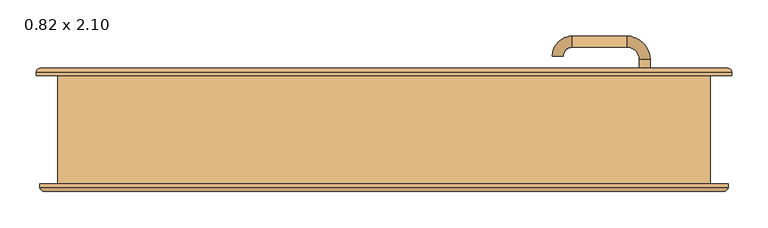
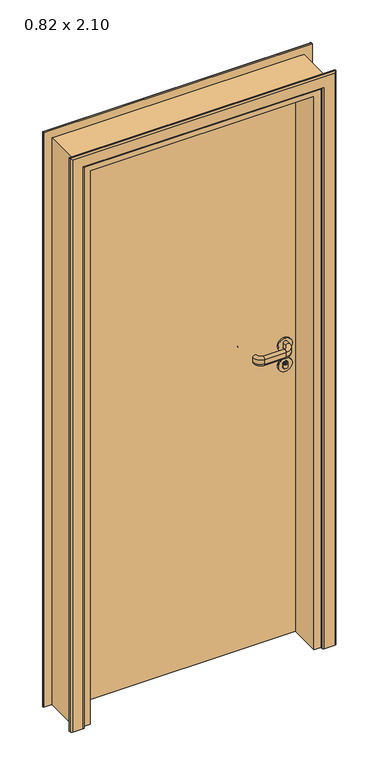
"""IFC4 building model written with IfcOpenShell, lengths in millimetres: door geometry, CC_PORTA ABRIR_1 FOLHA LISA : 0.82 x 2.10."""

from ifc_helpers import new_model, si_unit, point, frame, frame_2d, origin, origin_with_axes, place, context, project, spatial, polyline, circle_curve, ellipse_curve, trimmed, segment, composite_curve, outline, extrude, faceted_brep, source, transform, mapped, element, save
from ifc_brep_helpers import plane_surface, cylinder_surface, revolved_surface, advanced_brep


def door_0_82_x_2_10_9ce577dd(model_context):
    return source(origin(), model_context, "Body", "SolidModel", [
        advanced_brep(
        [(352.5, 40.0, 1091.5062746), (352.5, 40.0, 1108.3826844), (367.5, 40.0, 1108.3826844), (367.5, 40.0, 1091.5062746), (367.5, 18.0, 1108.3826844), (367.5, 18.0, 1091.5062746), (352.5, 18.0, 1091.5062746), (352.5, 18.0, 1108.3826844), (335.0, -14.5, 1108.3826844), (260.0, -14.5, 1108.3826844), (260.0, -14.5, 1091.5062746), (335.0, -14.5, 1091.5062746), (335.0, 0.5, 1091.5062746), (260.0, 0.5, 1091.5062746), (260.0, 0.5, 1108.3826844), (335.0, 0.5, 1108.3826844), (247.5, 13.0, 1091.5062746), (232.5, 13.0, 1091.5062746), (232.5, 13.0, 1108.3826844), (247.5, 13.0, 1108.3826844)],
        [
            (0, 1),
            (1, 2, circle_curve(frame((360.0, 40.0, 1108.3826844), z_axis=(0.0, 1.0, 0.0), x_axis=(0.0, 0.0, 1.0)), 7.5)),
            (2, 3),
            (3, 0, circle_curve(frame((360.0, 40.0, 1091.5062746), z_axis=(0.0, 1.0, 0.0), x_axis=(0.0, 0.0, 1.0)), 7.5)),
            (2, 4),
            (4, 5),
            (5, 3),
            (0, 6),
            (6, 7),
            (7, 1),
            (8, 9),
            (9, 10),
            (10, 11),
            (11, 8),
            (12, 13),
            (13, 14),
            (14, 15),
            (15, 12),
            (5, 6, circle_curve(frame((360.0, 18.0, 1091.5062746), z_axis=(0.0, 1.0, 0.0), x_axis=(0.0, 0.0, 1.0)), 7.5)),
            (7, 4, circle_curve(frame((360.0, 18.0, 1108.3826844), z_axis=(0.0, 1.0, 0.0), x_axis=(0.0, 0.0, 1.0)), 7.5)),
            (10, 13, circle_curve(frame((260.0, -7.0, 1091.5062746), z_axis=(1.0, 0.0, 0.0), x_axis=(0.0, 0.0, 1.0)), 7.5)),
            (12, 11, circle_curve(frame((335.0, -7.0, 1091.5062746), z_axis=(-1.0, 0.0, 0.0), x_axis=(0.0, 0.0, 1.0)), 7.5)),
            (14, 9, circle_curve(frame((260.0, -7.0, 1108.3826844), z_axis=(1.0, 0.0, 0.0), x_axis=(0.0, 0.0, 1.0)), 7.5)),
            (8, 15, circle_curve(frame((335.0, -7.0, 1108.3826844), z_axis=(-1.0, 0.0, 0.0), x_axis=(0.0, 0.0, 1.0)), 7.5)),
            (12, 6, circle_curve(frame((335.0, 18.0, 1091.5062746), z_axis=(0.0, 0.0, 1.0), x_axis=(1.0, 0.0, 0.0)), 17.5)),
            (5, 11, circle_curve(frame((335.0, 18.0, 1091.5062746), z_axis=(0.0, 0.0, -1.0), x_axis=(1.0, 0.0, 0.0)), 32.5)),
            (4, 8, circle_curve(frame((335.0, 18.0, 1108.3826844), z_axis=(0.0, 0.0, -1.0), x_axis=(1.0, 0.0, 0.0)), 32.5)),
            (7, 15, circle_curve(frame((335.0, 18.0, 1108.3826844), z_axis=(0.0, 0.0, -1.0), x_axis=(1.0, 0.0, 0.0)), 17.5)),
            (16, 17, circle_curve(frame((240.0, 13.0, 1091.5062746), z_axis=(0.0, 1.0, 0.0), x_axis=(0.0, 0.0, 1.0)), 7.5)),
            (17, 18),
            (18, 19, circle_curve(frame((240.0, 13.0, 1108.3826844), z_axis=(0.0, 1.0, 0.0), x_axis=(0.0, 0.0, 1.0)), 7.5)),
            (19, 16),
            (16, 13, circle_curve(frame((260.0, 13.0, 1091.5062746), z_axis=(0.0, 0.0, 1.0), x_axis=(0.0, -1.0, 0.0)), 12.5)),
            (10, 17, circle_curve(frame((260.0, 13.0, 1091.5062746), z_axis=(0.0, 0.0, -1.0), x_axis=(0.0, -1.0, 0.0)), 27.5)),
            (9, 18, circle_curve(frame((260.0, 13.0, 1108.3826844), z_axis=(0.0, 0.0, -1.0), x_axis=(0.0, -1.0, 0.0)), 27.5)),
            (14, 19, circle_curve(frame((260.0, 13.0, 1108.3826844), z_axis=(0.0, 0.0, -1.0), x_axis=(0.0, -1.0, 0.0)), 12.5)),
        ],
        [
            plane_surface(frame((360.0, 40.0, 1099.9444795), z_axis=(0.0, 1.0, 0.0), x_axis=(0.0, 0.0, 1.0))),
            plane_surface(frame((367.5, 40.0, 1091.5062746), z_axis=(1.0, 0.0, 0.0), x_axis=(0.0, -1.0, 0.0))),
            plane_surface(frame((352.5, 40.0, 1108.3826844), z_axis=(-1.0, 0.0, 0.0), x_axis=(0.0, -1.0, 0.0))),
            plane_surface(frame((335.0, -14.5, 1091.5062746), z_axis=(0.0, -1.0, 0.0), x_axis=(-1.0, 0.0, 0.0))),
            plane_surface(frame((335.0, 0.5, 1108.3826844), z_axis=(0.0, 1.0, 0.0), x_axis=(-1.0, 0.0, 0.0))),
            cylinder_surface(frame((360.0, 40.0, 1091.5062746), z_axis=(0.0, 1.0, 0.0), x_axis=(0.0, 0.0, 1.0)), 7.5),
            cylinder_surface(frame((360.0, 40.0, 1108.3826844), z_axis=(0.0, 1.0, 0.0), x_axis=(0.0, 0.0, 1.0)), 7.5),
            cylinder_surface(frame((335.0, -7.0, 1091.5062746), z_axis=(1.0, 0.0, 0.0), x_axis=(0.0, 0.0, 1.0)), 7.5),
            cylinder_surface(frame((335.0, -7.0, 1108.3826844), z_axis=(1.0, 0.0, 0.0), x_axis=(0.0, 0.0, 1.0)), 7.5),
            revolved_surface(trimmed(ellipse_curve(frame((360.0, 18.0, 1091.5062746), z_axis=(0.0, -1.0, 0.0), x_axis=(0.0, 0.0, 1.0)), 7.5, 7.5), [point((352.5, 18.0, 1091.5062746))], [point((367.5, 18.0, 1091.5062746))], True, "CARTESIAN"), (335.0, 18.0, 1099.9444795), (0.0, 0.0, 1.0)),
            cylinder_surface(frame((335.0, 18.0, 1099.9444795), z_axis=(0.0, 0.0, 1.0), x_axis=(1.0, 0.0, 0.0)), 32.5),
            revolved_surface(trimmed(ellipse_curve(frame((360.0, 18.0, 1108.3826844), z_axis=(0.0, -1.0, 0.0), x_axis=(0.0, 0.0, 1.0)), 7.5, 7.5), [point((367.5, 18.0, 1108.3826844))], [point((352.5, 18.0, 1108.3826844))], True, "CARTESIAN"), (335.0, 18.0, 1099.9444795), (0.0, 0.0, 1.0)),
            revolved_surface(polyline([(352.5, 18.0, 1108.3826844), (352.5, 18.0, 1091.5062746)]), (335.0, 18.0, 1099.9444795), (0.0, 0.0, 1.0)),
            plane_surface(frame((240.0, 13.0, 1099.9444795), z_axis=(0.0, 1.0, 0.0), x_axis=(0.0, 0.0, 1.0))),
            revolved_surface(trimmed(ellipse_curve(frame((260.0, -7.0, 1091.5062746), z_axis=(-1.0, 0.0, 0.0), x_axis=(0.0, 0.0, 1.0)), 7.5, 7.5), [point((260.0, 0.5, 1091.5062746))], [point((260.0, -14.5, 1091.5062746))], True, "CARTESIAN"), (260.0, 13.0, 1099.9444795), (0.0, 0.0, 1.0)),
            cylinder_surface(frame((260.0, 13.0, 1099.9444795), z_axis=(0.0, 0.0, 1.0), x_axis=(0.0, -1.0, 0.0)), 27.5),
            revolved_surface(trimmed(ellipse_curve(frame((260.0, -7.0, 1108.3826844), z_axis=(-1.0, 0.0, 0.0), x_axis=(0.0, 0.0, 1.0)), 7.5, 7.5), [point((260.0, -14.5, 1108.3826844))], [point((260.0, 0.5, 1108.3826844))], True, "CARTESIAN"), (260.0, 13.0, 1099.9444795), (0.0, 0.0, 1.0)),
            revolved_surface(polyline([(260.0, 0.5, 1108.3826844), (260.0, 0.5, 1091.5062746)]), (260.0, 13.0, 1099.9444795), (0.0, 0.0, 1.0)),
        ],
        [
            (0, [[1, 2, 3, 4]]),
            (1, [[5, 6, 7, -3]]),
            (2, [[8, 9, 10, -1]]),
            (3, [[11, 12, 13, 14]]),
            (4, [[15, 16, 17, 18]]),
            (5, [[-7, 19, -8, -4]]),
            (6, [[-10, 20, -5, -2]]),
            (7, [[-13, 21, -15, 22]]),
            (8, [[-17, 23, -11, 24]]),
            (9, [[-22, 25, -19, 26]]),
            (10, [[-14, -26, -6, 27]]),
            (11, [[-24, -27, -20, 28]]),
            (12, [[-18, -28, -9, -25]]),
            (13, [[29, 30, 31, 32]]),
            (14, [[-29, 33, -21, 34]]),
            (15, [[-30, -34, -12, 35]]),
            (16, [[-31, -35, -23, 36]]),
            (17, [[-32, -36, -16, -33]]),
        ],
    ),
        extrude(outline(polyline([(361.0, 40.0), (361.0, 30.9), (359.0, 30.9), (359.0, 40.0), (361.0, 40.0)])), frame((0.0, 0.0, 1027.9555433), z_axis=(0.0, 0.0, 1.0), x_axis=(1.0, 0.0, 0.0)), (0.0, 0.0, 1.0), 7.8071257),
        extrude(outline(composite_curve([segment(trimmed(circle_curve(frame_2d((1031.5611613, 360.0)), 5.0), [point((1036.5611613, 360.0))], [point((1026.5611613, 360.0))], False, "CARTESIAN"), True, "CONTINUOUS"), segment(trimmed(circle_curve(frame_2d((1031.5611613, 360.0)), 5.0), [point((1026.5611613, 360.0))], [point((1036.5611613, 360.0))], False, "CARTESIAN"), True, "CONTINUOUS")], self_intersect=False), holes=[polyline([(1035.7626689, 361.0), (1027.9555433, 361.0), (1027.9555433, 359.0), (1035.7626689, 359.0), (1035.7626689, 361.0)])]), frame((0.0, 30.0, 0.0), z_axis=(0.0, 1.0, 0.0), x_axis=(0.0, 0.0, 1.0)), (0.0, 0.0, 1.0), 10.0),
        extrude(outline(composite_curve([segment(polyline([(1033.4817325, 352.5), (1016.4817325, 352.5)]), True, "CONTINUOUS"), segment(trimmed(circle_curve(frame_2d((1016.4817325, 356.5)), 4.0), [point((1016.4817325, 352.5))], [point((1012.4817325, 356.5))], False, "CARTESIAN"), True, "CONTINUOUS"), segment(polyline([(1012.4817325, 356.5), (1012.4817325, 363.5)]), True, "CONTINUOUS"), segment(trimmed(circle_curve(frame_2d((1016.4817325, 363.5)), 4.0), [point((1012.4817325, 363.5))], [point((1016.4817325, 367.5))], False, "CARTESIAN"), True, "CONTINUOUS"), segment(polyline([(1016.4817325, 367.5), (1033.4817325, 367.5)]), True, "CONTINUOUS"), segment(trimmed(circle_curve(frame_2d((1033.4817325, 363.5)), 4.0), [point((1033.4817325, 367.5))], [point((1037.4817325, 363.5))], False, "CARTESIAN"), True, "CONTINUOUS"), segment(polyline([(1037.4817325, 363.5), (1037.4817325, 356.5)]), True, "CONTINUOUS"), segment(trimmed(circle_curve(frame_2d((1033.4817325, 356.5)), 4.0), [point((1037.4817325, 356.5))], [point((1033.4817325, 352.5))], False, "CARTESIAN"), True, "CONTINUOUS")], self_intersect=False)), frame((0.0, 31.0, 0.0), z_axis=(0.0, 1.0, 0.0), x_axis=(0.0, 0.0, 1.0)), (0.0, 0.0, 1.0), 9.0),
        extrude(outline(composite_curve([segment(trimmed(circle_curve(frame_2d((1099.9444795, 360.0)), 25.0), [point((1124.9444795, 360.0))], [point((1074.9444795, 360.0))], False, "CARTESIAN"), True, "CONTINUOUS"), segment(trimmed(circle_curve(frame_2d((1099.9444795, 360.0)), 25.0), [point((1074.9444795, 360.0))], [point((1124.9444795, 360.0))], False, "CARTESIAN"), True, "CONTINUOUS")], self_intersect=False)), frame((0.0, 34.0, 0.0), z_axis=(0.0, 1.0, 0.0), x_axis=(0.0, 0.0, 1.0)), (0.0, 0.0, 1.0), 6.0),
        extrude(outline(composite_curve([segment(trimmed(circle_curve(frame_2d((1024.9444795, 360.0)), 25.0), [point((1049.9444795, 360.0))], [point((999.9444795, 360.0))], False, "CARTESIAN"), True, "CONTINUOUS"), segment(trimmed(circle_curve(frame_2d((1024.9444795, 360.0)), 25.0), [point((999.9444795, 360.0))], [point((1049.9444795, 360.0))], False, "CARTESIAN"), True, "CONTINUOUS")], self_intersect=False), holes=[composite_curve([segment(trimmed(circle_curve(frame_2d((1033.4817325, 363.5)), 4.0), [point((1037.4817325, 363.5))], [point((1033.4817325, 367.5))], True, "CARTESIAN"), True, "CONTINUOUS"), segment(polyline([(1033.4817325, 367.5), (1016.4817325, 367.5)]), True, "CONTINUOUS"), segment(trimmed(circle_curve(frame_2d((1016.4817325, 363.5)), 4.0), [point((1016.4817325, 367.5))], [point((1012.4817325, 363.5))], True, "CARTESIAN"), True, "CONTINUOUS"), segment(polyline([(1012.4817325, 363.5), (1012.4817325, 356.5)]), True, "CONTINUOUS"), segment(trimmed(circle_curve(frame_2d((1016.4817325, 356.5)), 4.0), [point((1012.4817325, 356.5))], [point((1016.4817325, 352.5))], True, "CARTESIAN"), True, "CONTINUOUS"), segment(polyline([(1016.4817325, 352.5), (1033.4817325, 352.5)]), True, "CONTINUOUS"), segment(trimmed(circle_curve(frame_2d((1033.4817325, 356.5)), 4.0), [point((1033.4817325, 352.5))], [point((1037.4817325, 356.5))], True, "CARTESIAN"), True, "CONTINUOUS"), segment(polyline([(1037.4817325, 356.5), (1037.4817325, 363.5)]), True, "CONTINUOUS")], self_intersect=False)]), frame((0.0, 34.0, 0.0), z_axis=(0.0, 1.0, 0.0), x_axis=(0.0, 0.0, 1.0)), (0.0, 0.0, 1.0), 6.0),
        extrude(outline(polyline([(361.0, 84.1), (361.0, 75.0), (359.0, 75.0), (359.0, 84.1), (361.0, 84.1)])), frame((0.0, 0.0, 1027.9555433), z_axis=(0.0, 0.0, 1.0), x_axis=(1.0, 0.0, 0.0)), (0.0, 0.0, 1.0), 7.8071257),
        advanced_brep(
        [(360.0, 85.0, 1036.5611613), (360.0, 85.0, 1026.5611613), (361.0, 85.0, 1035.7626689), (359.0, 85.0, 1035.7626689), (359.0, 85.0, 1027.9555433), (361.0, 85.0, 1027.9555433), (360.0, 75.0, 1049.9444795), (360.0, 75.0, 999.9444795), (360.0, 84.0, 1026.5611613), (360.0, 84.0, 1036.5611613), (361.0, 84.0, 1027.9555433), (361.0, 84.0, 1035.7626689), (359.0, 84.0, 1027.9555433), (359.0, 84.0, 1035.7626689), (352.5, 84.0, 1033.4817325), (356.5, 84.0, 1037.4817325), (363.5, 84.0, 1037.4817325), (367.5, 84.0, 1033.4817325), (367.5, 84.0, 1016.4817325), (363.5, 84.0, 1012.4817325), (356.5, 84.0, 1012.4817325), (352.5, 84.0, 1016.4817325), (352.5, 81.0, 1016.4817325), (352.5, 81.0, 1033.4817325), (356.5, 81.0, 1012.4817325), (363.5, 81.0, 1012.4817325), (367.5, 81.0, 1016.4817325), (367.5, 81.0, 1033.4817325), (363.5, 81.0, 1037.4817325), (356.5, 81.0, 1037.4817325), (360.0, 81.0, 1049.9444795), (360.0, 81.0, 999.9444795)],
        [
            (0, 1, circle_curve(frame((360.0, 85.0, 1031.5611613), z_axis=(0.0, 1.0, 0.0), x_axis=(0.0, 0.0, -1.0)), 5.0)),
            (1, 0, circle_curve(frame((360.0, 85.0, 1031.5611613), z_axis=(0.0, 1.0, 0.0), x_axis=(0.0, 0.0, -1.0)), 5.0)),
            (2, 3),
            (3, 4),
            (4, 5),
            (5, 2),
            (6, 7, circle_curve(frame((360.0, 75.0, 1024.9444795), z_axis=(0.0, -1.0, 0.0), x_axis=(0.0, 0.0, -1.0)), 25.0)),
            (7, 6, circle_curve(frame((360.0, 75.0, 1024.9444795), z_axis=(0.0, -1.0, 0.0), x_axis=(0.0, 0.0, -1.0)), 25.0)),
            (1, 8),
            (8, 9, circle_curve(frame((360.0, 84.0, 1031.5611613), z_axis=(0.0, 1.0, 0.0), x_axis=(0.0, 0.0, -1.0)), 5.0)),
            (9, 0),
            (9, 8, circle_curve(frame((360.0, 84.0, 1031.5611613), z_axis=(0.0, 1.0, 0.0), x_axis=(0.0, 0.0, -1.0)), 5.0)),
            (5, 10),
            (10, 11),
            (11, 2),
            (4, 12),
            (12, 10),
            (3, 13),
            (13, 12),
            (11, 13),
            (14, 15, circle_curve(frame((356.5, 84.0, 1033.4817325), z_axis=(0.0, 1.0, 0.0), x_axis=(0.0, 0.0, -1.0)), 4.0)),
            (15, 16),
            (16, 17, circle_curve(frame((363.5, 84.0, 1033.4817325), z_axis=(0.0, 1.0, 0.0), x_axis=(0.0, 0.0, -1.0)), 4.0)),
            (17, 18),
            (18, 19, circle_curve(frame((363.5, 84.0, 1016.4817325), z_axis=(0.0, 1.0, 0.0), x_axis=(0.0, 0.0, -1.0)), 4.0)),
            (19, 20),
            (20, 21, circle_curve(frame((356.5, 84.0, 1016.4817325), z_axis=(0.0, 1.0, 0.0), x_axis=(0.0, 0.0, -1.0)), 4.0)),
            (21, 14),
            (21, 22),
            (22, 23),
            (23, 14),
            (20, 24),
            (24, 22, circle_curve(frame((356.5, 81.0, 1016.4817325), z_axis=(0.0, 1.0, 0.0), x_axis=(0.0, 0.0, -1.0)), 4.0)),
            (19, 25),
            (25, 24),
            (18, 26),
            (26, 25, circle_curve(frame((363.5, 81.0, 1016.4817325), z_axis=(0.0, 1.0, 0.0), x_axis=(0.0, 0.0, -1.0)), 4.0)),
            (17, 27),
            (27, 26),
            (16, 28),
            (28, 27, circle_curve(frame((363.5, 81.0, 1033.4817325), z_axis=(0.0, 1.0, 0.0), x_axis=(0.0, 0.0, -1.0)), 4.0)),
            (15, 29),
            (29, 28),
            (23, 29, circle_curve(frame((356.5, 81.0, 1033.4817325), z_axis=(0.0, 1.0, 0.0), x_axis=(0.0, 0.0, -1.0)), 4.0)),
            (30, 31, circle_curve(frame((360.0, 81.0, 1024.9444795), z_axis=(0.0, 1.0, 0.0), x_axis=(0.0, 0.0, -1.0)), 25.0)),
            (31, 30, circle_curve(frame((360.0, 81.0, 1024.9444795), z_axis=(0.0, 1.0, 0.0), x_axis=(0.0, 0.0, -1.0)), 25.0)),
            (31, 7),
            (6, 30),
        ],
        [
            plane_surface(frame((360.0, 85.0, 1026.5611613), z_axis=(0.0, 1.0, 0.0), x_axis=(1.0, 0.0, 0.0))),
            plane_surface(frame((360.0, 75.0, 1026.5611613), z_axis=(0.0, -1.0, 0.0), x_axis=(-1.0, 0.0, 0.0))),
            cylinder_surface(frame((360.0, 75.0, 1031.5611613), z_axis=(0.0, 1.0, 0.0), x_axis=(0.0, 0.0, -1.0)), 5.0),
            plane_surface(frame((361.0, 85.0, 1035.7626689), z_axis=(-1.0, 0.0, 0.0), x_axis=(0.0, -1.0, 0.0))),
            plane_surface(frame((361.0, 85.0, 1027.9555433), z_axis=(0.0, 0.0, 1.0), x_axis=(0.0, -1.0, 0.0))),
            plane_surface(frame((359.0, 85.0, 1027.9555433), z_axis=(1.0, 0.0, 0.0), x_axis=(0.0, -1.0, 0.0))),
            plane_surface(frame((359.0, 85.0, 1035.7626689), z_axis=(0.0, 0.0, -1.0), x_axis=(0.0, -1.0, 0.0))),
            plane_surface(frame((352.5, 84.0, 1016.4817325), z_axis=(0.0, 1.0, 0.0), x_axis=(0.0, 0.0, -1.0))),
            plane_surface(frame((352.5, 84.0, 1033.4817325), z_axis=(-1.0, 0.0, 0.0), x_axis=(0.0, -1.0, 0.0))),
            cylinder_surface(frame((356.5, 75.0, 1016.4817325), z_axis=(0.0, 1.0, 0.0), x_axis=(0.0, 0.0, -1.0)), 4.0),
            plane_surface(frame((356.5, 84.0, 1012.4817325), z_axis=(0.0, 0.0, -1.0), x_axis=(0.0, -1.0, 0.0))),
            cylinder_surface(frame((363.5, 75.0, 1016.4817325), z_axis=(0.0, 1.0, 0.0), x_axis=(0.0, 0.0, -1.0)), 4.0),
            plane_surface(frame((367.5, 84.0, 1016.4817325), z_axis=(1.0, 0.0, 0.0), x_axis=(0.0, -1.0, 0.0))),
            cylinder_surface(frame((363.5, 75.0, 1033.4817325), z_axis=(0.0, 1.0, 0.0), x_axis=(0.0, 0.0, -1.0)), 4.0),
            plane_surface(frame((363.5, 84.0, 1037.4817325), z_axis=(0.0, 0.0, 1.0), x_axis=(0.0, -1.0, 0.0))),
            cylinder_surface(frame((356.5, 75.0, 1033.4817325), z_axis=(0.0, 1.0, 0.0), x_axis=(0.0, 0.0, -1.0)), 4.0),
            plane_surface(frame((360.0, 81.0, 1074.9444795), z_axis=(0.0, 1.0, 0.0), x_axis=(1.0, 0.0, 0.0))),
            cylinder_surface(frame((360.0, 75.0, 1024.9444795), z_axis=(0.0, 1.0, 0.0), x_axis=(0.0, 0.0, -1.0)), 25.0),
        ],
        [
            (0, [[1, 2], [3, 4, 5, 6]]),
            (1, [[7, 8]]),
            (2, [[9, 10, 11, -2]]),
            (2, [[-11, 12, -9, -1]]),
            (3, [[13, 14, 15, -6]]),
            (4, [[16, 17, -13, -5]]),
            (5, [[18, 19, -16, -4]]),
            (6, [[-15, 20, -18, -3]]),
            (7, [[-17, -19, -20, -14]]),
            (7, [[21, 22, 23, 24, 25, 26, 27, 28], [-12, -10]]),
            (8, [[29, 30, 31, -28]]),
            (9, [[32, 33, -29, -27]]),
            (10, [[34, 35, -32, -26]]),
            (11, [[36, 37, -34, -25]]),
            (12, [[38, 39, -36, -24]]),
            (13, [[40, 41, -38, -23]]),
            (14, [[42, 43, -40, -22]]),
            (15, [[-31, 44, -42, -21]]),
            (16, [[45, 46], [-33, -35, -37, -39, -41, -43, -44, -30]]),
            (17, [[47, -7, 48, -46]]),
            (17, [[-48, -8, -47, -45]]),
        ],
    ),
        advanced_brep(
        [(360.0, 75.0, 1124.9444795), (360.0, 75.0, 1074.9444795), (360.0, 81.0, 1124.9444795), (360.0, 81.0, 1074.9444795)],
        [
            (0, 1, circle_curve(frame((360.0, 75.0, 1099.9444795), z_axis=(0.0, -1.0, 0.0), x_axis=(0.0, 0.0, -1.0)), 25.0)),
            (1, 0, circle_curve(frame((360.0, 75.0, 1099.9444795), z_axis=(0.0, -1.0, 0.0), x_axis=(0.0, 0.0, -1.0)), 25.0)),
            (2, 3, circle_curve(frame((360.0, 81.0, 1099.9444795), z_axis=(0.0, 1.0, 0.0), x_axis=(0.0, 0.0, -1.0)), 25.0)),
            (3, 2, circle_curve(frame((360.0, 81.0, 1099.9444795), z_axis=(0.0, 1.0, 0.0), x_axis=(0.0, 0.0, -1.0)), 25.0)),
            (3, 1),
            (0, 2),
        ],
        [
            plane_surface(frame((360.0, 75.0, 1026.5611613), z_axis=(0.0, -1.0, 0.0), x_axis=(-1.0, 0.0, 0.0))),
            plane_surface(frame((360.0, 81.0, 1074.9444795), z_axis=(0.0, 1.0, 0.0), x_axis=(1.0, 0.0, 0.0))),
            cylinder_surface(frame((360.0, 75.0, 1099.9444795), z_axis=(0.0, 1.0, 0.0), x_axis=(0.0, 0.0, -1.0)), 25.0),
        ],
        [
            (0, [[1, 2]]),
            (1, [[3, 4]]),
            (2, [[5, -1, 6, -4]]),
            (2, [[-6, -2, -5, -3]]),
        ],
    ),
        advanced_brep(
        [(352.5, 75.0, 1108.4382049), (352.5, 75.0, 1091.5617951), (367.5, 75.0, 1091.5617951), (367.5, 75.0, 1108.4382049), (367.5, 97.0, 1091.5617951), (367.5, 97.0, 1108.4382049), (352.5, 97.0, 1108.4382049), (352.5, 97.0, 1091.5617951), (335.0, 129.5, 1091.5617951), (260.0, 129.5, 1091.5617951), (260.0, 129.5, 1108.4382049), (335.0, 129.5, 1108.4382049), (335.0, 114.5, 1108.4382049), (260.0, 114.5, 1108.4382049), (260.0, 114.5, 1091.5617951), (335.0, 114.5, 1091.5617951), (247.5, 102.0, 1108.4382049), (232.5, 102.0, 1108.4382049), (232.5, 102.0, 1091.5617951), (247.5, 102.0, 1091.5617951)],
        [
            (0, 1),
            (1, 2, circle_curve(frame((360.0, 75.0, 1091.5617951), z_axis=(0.0, -1.0, 0.0), x_axis=(-1.0, 0.0, 0.0)), 7.5)),
            (2, 3),
            (3, 0, circle_curve(frame((360.0, 75.0, 1108.4382049), z_axis=(0.0, -1.0, 0.0), x_axis=(-1.0, 0.0, 0.0)), 7.5)),
            (2, 4),
            (4, 5),
            (5, 3),
            (0, 6),
            (6, 7),
            (7, 1),
            (8, 9),
            (9, 10),
            (10, 11),
            (11, 8),
            (12, 13),
            (13, 14),
            (14, 15),
            (15, 12),
            (5, 6, circle_curve(frame((360.0, 97.0, 1108.4382049), z_axis=(0.0, -1.0, 0.0), x_axis=(-1.0, 0.0, 0.0)), 7.5)),
            (7, 4, circle_curve(frame((360.0, 97.0, 1091.5617951), z_axis=(0.0, -1.0, 0.0), x_axis=(-1.0, 0.0, 0.0)), 7.5)),
            (10, 13, circle_curve(frame((260.0, 122.0, 1108.4382049), z_axis=(1.0, 0.0, 0.0), x_axis=(0.0, -1.0, 0.0)), 7.5)),
            (12, 11, circle_curve(frame((335.0, 122.0, 1108.4382049), z_axis=(-1.0, 0.0, 0.0), x_axis=(0.0, -1.0, 0.0)), 7.5)),
            (14, 9, circle_curve(frame((260.0, 122.0, 1091.5617951), z_axis=(1.0, 0.0, 0.0), x_axis=(0.0, -1.0, 0.0)), 7.5)),
            (8, 15, circle_curve(frame((335.0, 122.0, 1091.5617951), z_axis=(-1.0, 0.0, 0.0), x_axis=(0.0, -1.0, 0.0)), 7.5)),
            (12, 6, circle_curve(frame((335.0, 97.0, 1108.4382049), z_axis=(0.0, 0.0, -1.0), x_axis=(1.0, 0.0, 0.0)), 17.5)),
            (5, 11, circle_curve(frame((335.0, 97.0, 1108.4382049), z_axis=(0.0, 0.0, 1.0), x_axis=(1.0, 0.0, 0.0)), 32.5)),
            (4, 8, circle_curve(frame((335.0, 97.0, 1091.5617951), z_axis=(0.0, 0.0, 1.0), x_axis=(1.0, 0.0, 0.0)), 32.5)),
            (7, 15, circle_curve(frame((335.0, 97.0, 1091.5617951), z_axis=(0.0, 0.0, 1.0), x_axis=(1.0, 0.0, 0.0)), 17.5)),
            (16, 17, circle_curve(frame((240.0, 102.0, 1108.4382049), z_axis=(0.0, -1.0, 0.0), x_axis=(1.0, 0.0, 0.0)), 7.5)),
            (17, 18),
            (18, 19, circle_curve(frame((240.0, 102.0, 1091.5617951), z_axis=(0.0, -1.0, 0.0), x_axis=(1.0, 0.0, 0.0)), 7.5)),
            (19, 16),
            (16, 13, circle_curve(frame((260.0, 102.0, 1108.4382049), z_axis=(0.0, 0.0, -1.0), x_axis=(0.0, 1.0, 0.0)), 12.5)),
            (10, 17, circle_curve(frame((260.0, 102.0, 1108.4382049), z_axis=(0.0, 0.0, 1.0), x_axis=(0.0, 1.0, 0.0)), 27.5)),
            (9, 18, circle_curve(frame((260.0, 102.0, 1091.5617951), z_axis=(0.0, 0.0, 1.0), x_axis=(0.0, 1.0, 0.0)), 27.5)),
            (14, 19, circle_curve(frame((260.0, 102.0, 1091.5617951), z_axis=(0.0, 0.0, 1.0), x_axis=(0.0, 1.0, 0.0)), 12.5)),
        ],
        [
            plane_surface(frame((360.0, 75.0, 1100.0), z_axis=(0.0, -1.0, 0.0), x_axis=(0.0, 0.0, -1.0))),
            plane_surface(frame((367.5, 75.0, 1108.4382049), z_axis=(1.0, 0.0, 0.0), x_axis=(0.0, 1.0, 0.0))),
            plane_surface(frame((352.5, 75.0, 1091.5617951), z_axis=(-1.0, 0.0, 0.0), x_axis=(0.0, 1.0, 0.0))),
            plane_surface(frame((335.0, 129.5, 1108.4382049), z_axis=(0.0, 1.0, 0.0), x_axis=(-1.0, 0.0, 0.0))),
            plane_surface(frame((335.0, 114.5, 1091.5617951), z_axis=(0.0, -1.0, 0.0), x_axis=(-1.0, 0.0, 0.0))),
            cylinder_surface(frame((360.0, 75.0, 1108.4382049), z_axis=(0.0, -1.0, 0.0), x_axis=(-1.0, 0.0, 0.0)), 7.5),
            cylinder_surface(frame((360.0, 75.0, 1091.5617951), z_axis=(0.0, -1.0, 0.0), x_axis=(-1.0, 0.0, 0.0)), 7.5),
            cylinder_surface(frame((335.0, 122.0, 1108.4382049), z_axis=(1.0, 0.0, 0.0), x_axis=(0.0, -1.0, 0.0)), 7.5),
            cylinder_surface(frame((335.0, 122.0, 1091.5617951), z_axis=(1.0, 0.0, 0.0), x_axis=(0.0, -1.0, 0.0)), 7.5),
            revolved_surface(trimmed(ellipse_curve(frame((360.0, 97.0, 1108.4382049), z_axis=(0.0, 1.0, 0.0), x_axis=(-1.0, 0.0, 0.0)), 7.5, 7.5), [point((352.5, 97.0, 1108.4382049))], [point((367.5, 97.0, 1108.4382049))], True, "CARTESIAN"), (335.0, 97.0, 1100.0), (0.0, 0.0, -1.0)),
            cylinder_surface(frame((335.0, 97.0, 1100.0), z_axis=(0.0, 0.0, -1.0), x_axis=(1.0, 0.0, 0.0)), 32.5),
            revolved_surface(trimmed(ellipse_curve(frame((360.0, 97.0, 1091.5617951), z_axis=(0.0, 1.0, 0.0), x_axis=(-1.0, 0.0, 0.0)), 7.5, 7.5), [point((367.5, 97.0, 1091.5617951))], [point((352.5, 97.0, 1091.5617951))], True, "CARTESIAN"), (335.0, 97.0, 1100.0), (0.0, 0.0, -1.0)),
            revolved_surface(polyline([(352.5, 97.0, 1091.5617951), (352.5, 97.0, 1108.4382049)]), (335.0, 97.0, 1100.0), (0.0, 0.0, -1.0)),
            plane_surface(frame((240.0, 102.0, 1100.0), z_axis=(0.0, -1.0, 0.0), x_axis=(0.0, 0.0, -1.0))),
            revolved_surface(trimmed(ellipse_curve(frame((260.0, 122.0, 1108.4382049), z_axis=(-1.0, 0.0, 0.0), x_axis=(0.0, -1.0, 0.0)), 7.5, 7.5), [point((260.0, 114.5, 1108.4382049))], [point((260.0, 129.5, 1108.4382049))], True, "CARTESIAN"), (260.0, 102.0, 1100.0), (0.0, 0.0, -1.0)),
            cylinder_surface(frame((260.0, 102.0, 1100.0), z_axis=(0.0, 0.0, -1.0), x_axis=(0.0, 1.0, 0.0)), 27.5),
            revolved_surface(trimmed(ellipse_curve(frame((260.0, 122.0, 1091.5617951), z_axis=(-1.0, 0.0, 0.0), x_axis=(0.0, -1.0, 0.0)), 7.5, 7.5), [point((260.0, 129.5, 1091.5617951))], [point((260.0, 114.5, 1091.5617951))], True, "CARTESIAN"), (260.0, 102.0, 1100.0), (0.0, 0.0, -1.0)),
            revolved_surface(polyline([(260.0, 114.5, 1091.5617951), (260.0, 114.5, 1108.4382049)]), (260.0, 102.0, 1100.0), (0.0, 0.0, -1.0)),
        ],
        [
            (0, [[1, 2, 3, 4]]),
            (1, [[5, 6, 7, -3]]),
            (2, [[8, 9, 10, -1]]),
            (3, [[11, 12, 13, 14]]),
            (4, [[15, 16, 17, 18]]),
            (5, [[-7, 19, -8, -4]]),
            (6, [[-10, 20, -5, -2]]),
            (7, [[-13, 21, -15, 22]]),
            (8, [[-17, 23, -11, 24]]),
            (9, [[-22, 25, -19, 26]]),
            (10, [[-14, -26, -6, 27]]),
            (11, [[-24, -27, -20, 28]]),
            (12, [[-18, -28, -9, -25]]),
            (13, [[29, 30, 31, 32]]),
            (14, [[-29, 33, -21, 34]]),
            (15, [[-30, -34, -12, 35]]),
            (16, [[-31, -35, -23, 36]]),
            (17, [[-32, -36, -16, -33]]),
        ],
    ),
        extrude(outline(polyline([(410.0, 75.0), (410.0, 40.0), (-410.0, 40.0), (-410.0, 75.0), (410.0, 75.0)])), origin_with_axes(), (0.0, 0.0, 1.0), 2100.0),
        advanced_brep(
        [(-430.5, -85.0, 0.0), (-469.500573, -85.0, 0.0), (-475.0, -79.500573, 0.0), (-475.0, -75.0, 0.0), (-425.0, -75.0, 0.0), (-425.0, -79.5, 0.0), (-425.0, -79.5, 2115.0), (-430.5, -85.0, 2120.5), (-425.0, -75.0, 2115.0), (-475.0, -75.0, 2165.0), (475.0, -75.0, 2165.0), (475.0, -75.0, 0.0), (425.0, -75.0, 0.0), (425.0, -75.0, 2115.0), (-475.0, -79.500573, 2165.0), (-469.500573, -85.0, 2159.500573), (430.5, -85.0, 2120.5), (430.5, -85.0, 0.0), (469.500573, -85.0, 0.0), (469.500573, -85.0, 2159.500573), (425.0, -79.5, 0.0), (425.0, -79.5, 2115.0), (475.0, -79.500573, 0.0), (475.0, -79.500573, 2165.0)],
        [
            (0, 1),
            (1, 2, circle_curve(frame((-469.500573, -79.500573, 0.0), z_axis=(0.0, 0.0, -1.0), x_axis=(0.0, -1.0, 0.0)), 5.499427)),
            (2, 3),
            (3, 4),
            (4, 5),
            (5, 0, circle_curve(frame((-430.5, -79.5, 0.0), z_axis=(0.0, 0.0, -1.0), x_axis=(0.0, -1.0, 0.0)), 5.5)),
            (5, 6),
            (6, 7, ellipse_curve(frame((-430.5, -79.5, 2120.5), z_axis=(-0.7071067811865475, 0.0, -0.7071067811865476), x_axis=(0.7071067811865476, 0.0, -0.7071067811865474)), 7.7781746, 5.5)),
            (7, 0),
            (4, 8),
            (8, 6),
            (3, 9),
            (9, 10),
            (10, 11),
            (11, 12),
            (12, 13),
            (13, 8),
            (2, 14),
            (14, 9),
            (1, 15),
            (15, 14, ellipse_curve(frame((-469.500573, -79.500573, 2159.500573), z_axis=(-0.7071067811865475, 0.0, -0.7071067811865476), x_axis=(0.7071067811865476, 0.0, -0.7071067811865474)), 7.7773642, 5.499427)),
            (7, 16),
            (16, 17),
            (17, 18),
            (18, 19),
            (19, 15),
            (12, 20),
            (20, 21),
            (21, 13),
            (17, 20, circle_curve(frame((430.5, -79.5, 0.0), z_axis=(0.0, 0.0, -1.0), x_axis=(0.0, -1.0, 0.0)), 5.5)),
            (11, 22),
            (22, 18, circle_curve(frame((469.500573, -79.500573, 0.0), z_axis=(0.0, 0.0, -1.0), x_axis=(0.0, -1.0, 0.0)), 5.499427)),
            (23, 22),
            (10, 23),
            (23, 19, ellipse_curve(frame((469.500573, -79.500573, 2159.500573), z_axis=(0.7071067811865475, 0.0, -0.7071067811865475), x_axis=(0.7071067811865474, 0.0, 0.7071067811865477)), 7.7773642, 5.499427)),
            (16, 21, ellipse_curve(frame((430.5, -79.5, 2120.5), z_axis=(0.7071067811865475, 0.0, -0.7071067811865475), x_axis=(0.7071067811865474, 0.0, 0.7071067811865477)), 7.7781746, 5.5)),
            (6, 21),
            (14, 23),
        ],
        [
            plane_surface(frame((-450.0, -75.0, 0.0), z_axis=(0.0, 0.0, -1.0), x_axis=(-1.0, 0.0, 0.0))),
            cylinder_surface(frame((-430.5, -79.5, 0.0), z_axis=(0.0, 0.0, -1.0), x_axis=(0.0, -1.0, 0.0)), 5.5),
            plane_surface(frame((-425.0, -79.5, 0.0), z_axis=(1.0, 0.0, 0.0), x_axis=(0.0, 0.0, 1.0))),
            plane_surface(frame((-425.0, -75.0, 0.0), z_axis=(0.0, 1.0, 0.0), x_axis=(0.0, 0.0, 1.0))),
            plane_surface(frame((-475.0, -75.0, 0.0), z_axis=(-1.0, 0.0, 0.0), x_axis=(0.0, 0.0, 1.0))),
            cylinder_surface(frame((-469.500573, -79.500573, 0.0), z_axis=(0.0, 0.0, -1.0), x_axis=(0.0, -1.0, 0.0)), 5.499427),
            plane_surface(frame((-469.500573, -85.0, 0.0), z_axis=(0.0, -1.0, 0.0), x_axis=(0.0, 0.0, 1.0))),
            plane_surface(frame((425.0, -79.5, 2115.0), z_axis=(-1.0, 0.0, 0.0), x_axis=(0.0, 0.0, -1.0))),
            plane_surface(frame((450.0, -75.0, 0.0), z_axis=(0.0, 0.0, -1.0), x_axis=(1.0, 0.0, 0.0))),
            plane_surface(frame((475.0, -75.0, 2165.0), z_axis=(1.0, 0.0, 0.0), x_axis=(0.0, 0.0, -1.0))),
            cylinder_surface(frame((469.500573, -79.500573, 2140.0), z_axis=(0.0, 0.0, 1.0), x_axis=(0.0, -1.0, 0.0)), 5.499427),
            cylinder_surface(frame((430.5, -79.5, 2140.0), z_axis=(0.0, 0.0, 1.0), x_axis=(0.0, -1.0, 0.0)), 5.5),
            cylinder_surface(frame((-450.0, -79.5, 2120.5), z_axis=(-1.0, 0.0, 0.0), x_axis=(0.0, -1.0, 0.0)), 5.5),
            plane_surface(frame((-425.0, -79.5, 2115.0), z_axis=(0.0, 0.0, -1.0), x_axis=(1.0, 0.0, 0.0))),
            plane_surface(frame((-475.0, -75.0, 2165.0), z_axis=(0.0, 0.0, 1.0), x_axis=(1.0, 0.0, 0.0))),
            cylinder_surface(frame((-450.0, -79.500573, 2159.500573), z_axis=(-1.0, 0.0, 0.0), x_axis=(0.0, -1.0, 0.0)), 5.499427),
        ],
        [
            (0, [[1, 2, 3, 4, 5, 6]]),
            (1, [[7, 8, 9, -6]]),
            (2, [[10, 11, -7, -5]]),
            (3, [[12, 13, 14, 15, 16, 17, -10, -4]]),
            (4, [[18, 19, -12, -3]]),
            (5, [[20, 21, -18, -2]]),
            (6, [[-9, 22, 23, 24, 25, 26, -20, -1]]),
            (7, [[-16, 27, 28, 29]]),
            (8, [[30, -27, -15, 31, 32, -24]]),
            (9, [[33, -31, -14, 34]]),
            (10, [[-25, -32, -33, 35]]),
            (11, [[-28, -30, -23, 36]]),
            (12, [[37, -36, -22, -8]]),
            (13, [[-17, -29, -37, -11]]),
            (14, [[38, -34, -13, -19]]),
            (15, [[-26, -35, -38, -21]]),
        ],
    ),
        advanced_brep(
        [(-430.0, 75.0, 0.0), (-480.0, 75.0, 0.0), (-480.0, 79.5, 0.0), (-474.5, 85.0, 0.0), (-435.5, 85.0, 0.0), (-430.0, 79.5, 0.0), (-430.0, 79.5, 2120.0), (-430.0, 75.0, 2120.0), (-435.5, 85.0, 2125.5), (-474.5, 85.0, 2164.5), (474.5, 85.0, 2164.5), (474.5, 85.0, 0.0), (435.5, 85.0, 0.0), (435.5, 85.0, 2125.5), (-480.0, 79.5, 2170.0), (-480.0, 75.0, 2170.0), (430.0, 75.0, 2120.0), (430.0, 75.0, 0.0), (480.0, 75.0, 0.0), (480.0, 75.0, 2170.0), (430.0, 79.5, 0.0), (430.0, 79.5, 2120.0), (480.0, 79.5, 0.0), (480.0, 79.5, 2170.0)],
        [
            (0, 1),
            (1, 2),
            (2, 3, circle_curve(frame((-474.5, 79.5, 0.0), z_axis=(0.0, 0.0, -1.0), x_axis=(0.0, -1.0, 0.0)), 5.5)),
            (3, 4),
            (4, 5, circle_curve(frame((-435.5, 79.5, 0.0), z_axis=(0.0, 0.0, -1.0), x_axis=(0.0, -1.0, 0.0)), 5.5)),
            (5, 0),
            (5, 6),
            (6, 7),
            (7, 0),
            (4, 8),
            (8, 6, ellipse_curve(frame((-435.5, 79.5, 2125.5), z_axis=(-0.7071067811865475, 0.0, -0.7071067811865476), x_axis=(0.7071067811865476, 0.0, -0.7071067811865474)), 7.7781746, 5.5)),
            (3, 9),
            (9, 10),
            (10, 11),
            (11, 12),
            (12, 13),
            (13, 8),
            (2, 14),
            (14, 9, ellipse_curve(frame((-474.5, 79.5, 2164.5), z_axis=(-0.7071067811865475, 0.0, -0.7071067811865476), x_axis=(0.7071067811865476, 0.0, -0.7071067811865474)), 7.7781746, 5.5)),
            (1, 15),
            (15, 14),
            (7, 16),
            (16, 17),
            (17, 18),
            (18, 19),
            (19, 15),
            (12, 20, circle_curve(frame((435.5, 79.5, 0.0), z_axis=(0.0, 0.0, 1.0), x_axis=(0.0, -1.0, 0.0)), 5.5)),
            (20, 21),
            (21, 13, ellipse_curve(frame((435.5, 79.5, 2125.5), z_axis=(0.7071067811865475, 0.0, -0.7071067811865475), x_axis=(0.7071067811865474, 0.0, 0.7071067811865477)), 7.7781746, 5.5)),
            (17, 20),
            (11, 22, circle_curve(frame((474.5, 79.5, 0.0), z_axis=(0.0, 0.0, -1.0), x_axis=(0.0, -1.0, 0.0)), 5.5)),
            (22, 18),
            (23, 22),
            (10, 23, ellipse_curve(frame((474.5, 79.5, 2164.5), z_axis=(0.7071067811865475, 0.0, -0.7071067811865475), x_axis=(0.7071067811865474, 0.0, 0.7071067811865477)), 7.7781746, 5.5)),
            (23, 19),
            (16, 21),
            (6, 21),
            (14, 23),
        ],
        [
            plane_surface(frame((-450.0, 75.0, 0.0), z_axis=(0.0, 0.0, -1.0), x_axis=(-1.0, 0.0, 0.0))),
            plane_surface(frame((-430.0, 75.0, 0.0), z_axis=(1.0, 0.0, 0.0), x_axis=(0.0, 0.0, 1.0))),
            cylinder_surface(frame((-435.5, 79.5, 0.0), z_axis=(0.0, 0.0, -1.0), x_axis=(0.0, -1.0, 0.0)), 5.5),
            plane_surface(frame((-435.5, 85.0, 0.0), z_axis=(0.0, 1.0, 0.0), x_axis=(0.0, 0.0, 1.0))),
            cylinder_surface(frame((-474.5, 79.5, 0.0), z_axis=(0.0, 0.0, -1.0), x_axis=(0.0, -1.0, 0.0)), 5.5),
            plane_surface(frame((-480.0, 79.5, 0.0), z_axis=(-1.0, 0.0, 0.0), x_axis=(0.0, 0.0, 1.0))),
            plane_surface(frame((-480.0, 75.0, 0.0), z_axis=(0.0, -1.0, 0.0), x_axis=(0.0, 0.0, 1.0))),
            cylinder_surface(frame((435.5, 79.5, 2140.0), z_axis=(0.0, 0.0, 1.0), x_axis=(0.0, -1.0, 0.0)), 5.5),
            plane_surface(frame((450.0, 75.0, 0.0), z_axis=(0.0, 0.0, -1.0), x_axis=(1.0, 0.0, 0.0))),
            cylinder_surface(frame((474.5, 79.5, 2140.0), z_axis=(0.0, 0.0, 1.0), x_axis=(0.0, -1.0, 0.0)), 5.5),
            plane_surface(frame((480.0, 79.5, 2170.0), z_axis=(1.0, 0.0, 0.0), x_axis=(0.0, 0.0, -1.0))),
            plane_surface(frame((430.0, 75.0, 2120.0), z_axis=(-1.0, 0.0, 0.0), x_axis=(0.0, 0.0, -1.0))),
            plane_surface(frame((-430.0, 75.0, 2120.0), z_axis=(0.0, 0.0, -1.0), x_axis=(1.0, 0.0, 0.0))),
            cylinder_surface(frame((-450.0, 79.5, 2125.5), z_axis=(-1.0, 0.0, 0.0), x_axis=(0.0, -1.0, 0.0)), 5.5),
            cylinder_surface(frame((-450.0, 79.5, 2164.5), z_axis=(-1.0, 0.0, 0.0), x_axis=(0.0, -1.0, 0.0)), 5.5),
            plane_surface(frame((-480.0, 79.5, 2170.0), z_axis=(0.0, 0.0, 1.0), x_axis=(1.0, 0.0, 0.0))),
        ],
        [
            (0, [[1, 2, 3, 4, 5, 6]]),
            (1, [[7, 8, 9, -6]]),
            (2, [[10, 11, -7, -5]]),
            (3, [[12, 13, 14, 15, 16, 17, -10, -4]]),
            (4, [[18, 19, -12, -3]]),
            (5, [[20, 21, -18, -2]]),
            (6, [[-9, 22, 23, 24, 25, 26, -20, -1]]),
            (7, [[-16, 27, 28, 29]]),
            (8, [[30, -27, -15, 31, 32, -24]]),
            (9, [[33, -31, -14, 34]]),
            (10, [[-25, -32, -33, 35]]),
            (11, [[-28, -30, -23, 36]]),
            (12, [[37, -36, -22, -8]]),
            (13, [[-17, -29, -37, -11]]),
            (14, [[38, -34, -13, -19]]),
            (15, [[-26, -35, -38, -21]]),
        ],
    ),
        faceted_brep([(-410.0, 40.0, 0.0), (-400.0, 40.0, 0.0), (-400.0, -75.0, 0.0), (-450.0, -75.0, 0.0), (-450.0, 75.0, 0.0), (-410.0, 75.0, 0.0), (-410.0, 75.0, 2100.0), (-410.0, 40.0, 2100.0), (-450.0, 75.0, 2140.0), (450.0, 75.0, 2140.0), (450.0, 75.0, 0.0), (410.0, 75.0, 0.0), (410.0, 75.0, 2100.0), (-450.0, -75.0, 2140.0), (-400.0, -75.0, 2090.0), (400.0, -75.0, 2090.0), (400.0, -75.0, 0.0), (450.0, -75.0, 0.0), (450.0, -75.0, 2140.0), (-400.0, 40.0, 2090.0), (410.0, 40.0, 2100.0), (410.0, 40.0, 0.0), (400.0, 40.0, 0.0), (400.0, 40.0, 2090.0)], [[[0, 1, 2, 3, 4, 5]], [[5, 6, 7, 0]], [[4, 8, 9, 10, 11, 12, 6, 5]], [[3, 13, 8, 4]], [[2, 14, 15, 16, 17, 18, 13, 3]], [[1, 19, 14, 2]], [[0, 7, 20, 21, 22, 23, 19, 1]], [[12, 11, 21, 20]], [[21, 11, 10, 17, 16, 22]], [[18, 17, 10, 9]], [[23, 22, 16, 15]], [[6, 12, 20, 7]], [[13, 18, 9, 8]], [[19, 23, 15, 14]]]),
    ])


if __name__ == "__main__":
    model = new_model("IFC4")
    model_context = context("Model", 3, world=origin())
    ifc_project = project(units=[si_unit("LENGTHUNIT", "METRE", prefix="MILLI")], contexts=[model_context])
    site = spatial("IfcSite", under=ifc_project)
    building = spatial("IfcBuilding", under=site)
    placement = place(None, origin())
    door_0_82_x_2_10_shape = door_0_82_x_2_10_9ce577dd(model_context)
    element("IfcDoor", 1, ObjectType="CC_PORTA ABRIR_1 FOLHA LISA : 0.82 x 2.10", at=placement, inside=building, context=model_context, shape_type="MappedRepresentation", body=[
        mapped(door_0_82_x_2_10_shape, transform((0.0, 0.0, 0.0), x_axis=(1.0, 0.0, 0.0), y_axis=(0.0, 1.0, 0.0), z_axis=(0.0, 0.0, 1.0))),
    ])
    save(model, "model.ifc")

# Revit data of these elements
# Type "CC_PORTA ABRIR_1 FOLHA LISA : 0.82 x 2.10"
#   Type Mark = "P6"
#   Site = "www.construir.arq.br"
#   Empresa = "Cursos Construir"
#   Description = "PORTA ABRIR 1 FOLHA LISA"
#   Criado Por = "Roberto Netto"
#   Analytic Construction = "<Nenhum>"
#   Atualizado por = "Rudemberg Eloi"
#   Rough Width = 0.90 m
#   Interna [instance default] = 0.00 m
#   Largura Guarnição Interna [instance default] = 0.05 m
#   Largura Guarnição Externa [instance default] = 0.05 m
#   Largura Folha [instance default] = 0.82 m
#   Externa [instance default] = 0.00 m
#   Extensão Lateral Esquerda [instance default] = 0.03 m
#   Extensão Lateral Direita [instance default] = 0.03 m
#   Extensão Frontal [instance default] = 0.03 m
#   Espessura Soleira [instance default] = 0.02 m
#   Espessura Guarnição Interna [instance default] = 0.01 m
#   Espessura Guarnição Externa [instance default] = 0.01 m
#   Espessura Folha [instance default] = 0.035 m
#   Espessura Batente [instance default] = 0.05 m
#   Eixo Rotação Folha [instance default] = 0.04 m
#   Deslocamento Maçaneta [instance default] = 0.05 m
#   Deslocamento Fechadura [instance default] = 0.05 m
#   Desloc (Interno) [instance default] = 0.02 m
#   Desloc (Externo) [instance default] = 0.025 m
#   Rough Height = 2.14 m
#   Altura Maçaneta [instance default] = 1.10 m
#   Altura Folha [instance default] = 2.10 m
#   Altura Fechadura [instance default] = 1.00 m
#   Height = 2.14 m
#   Width = 0.90 m
#   ----SOLEIRA---- [instance default] = 0.00 m
#   ----MAÇANETA/FECHADURA---- [instance default] = 0.00 m
#   ----GUARNIÇÃO---- [instance default] = 0.00 m
#   ----FOLHA---- [instance default] = 0.00 m
#   ----EXTENSÃO---- [instance default] = 0.00 m
#   ----BATENTE---- [instance default] = 0.00 m
#   Soleira Sem Extensão [instance default] = yes
#   Soleira Com Extensão [instance default] = no
#   Soleira [instance default] = yes
#   Maçaneta / Puxador [instance default] = yes
#   Guarnição Interna [instance default] = yes
#   Guarnição Externa [instance default] = yes
#   Fechadura Separada [instance default] = no
#   Bit [instance default] = no
#   Porcent. Exibição Batente Interno [instance default] = 50
#   Porcent. Exibição Batente Externo [instance default] = 50
#   Material Bit/Soleira = .GRANITO BRANCO ITAÚNAS
#   Material Espelho/Fixação = .AÇO INOXIDÁVEL ESCOVADO
#   Material Maçaneta/Puxador = .AÇO INOXIDÁVEL ESCOVADO
#   Material Guarnição Interna = .MADEIRA COM PINTURA ESMALTE BRANCO ACETINADO
#   Material Guarnição Externa = .MADEIRA COM PINTURA ESMALTE BRANCO ACETINADO
#   Material Folha = .MADEIRA COM PINTURA ESMALTE BRANCO ACETINADO
#   Material Fechadura = .AÇO INOXIDÁVEL ESCOVADO
#   Material Batente = .MADEIRA COM PINTURA ESMALTE BRANCO ACETINADO
#   Família Maçaneta [instance default] = element 1947931
#   Function = (empty or 0)
#   Wall Closure = (empty or 0)
# Element 1 (IfcDoor, "CC_PORTA ABRIR_1 FOLHA LISA : 0.82 x 2.10")
#   Materials on its faces: ".AÇO INOXIDÁVEL ESCOVADO", ".MADEIRA COM PINTURA ESMALTE BRANCO ACETINADO"
# Materials
#   ".GRANITO BRANCO ITAÚNAS": class ".CC_PEDRA REVEST.", colour RGB 202 195 174, transparency 0, Description = "Granito branco Itaúnas", Uso = "Pedra", Cost = 0
#   ".AÇO INOXIDÁVEL ESCOVADO": class "Metal", colour RGB 189 187 185, transparency 0, Description = "Stainless Steel 18/8, brushed finish", Cost = 0
#   ".MADEIRA COM PINTURA ESMALTE BRANCO ACETINADO": class ".CC_MADEIRAS", colour RGB 240 240 240, transparency 0, Description = "Madeira com pintura esmalte branco acetinado.", Cost = 0
